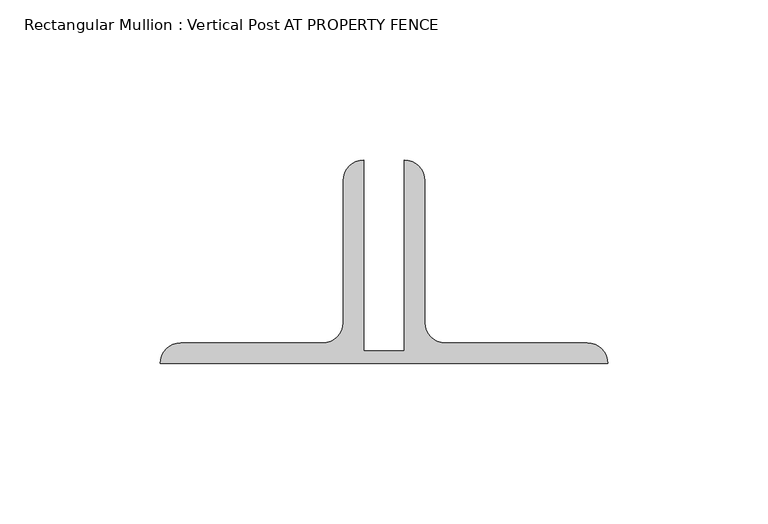
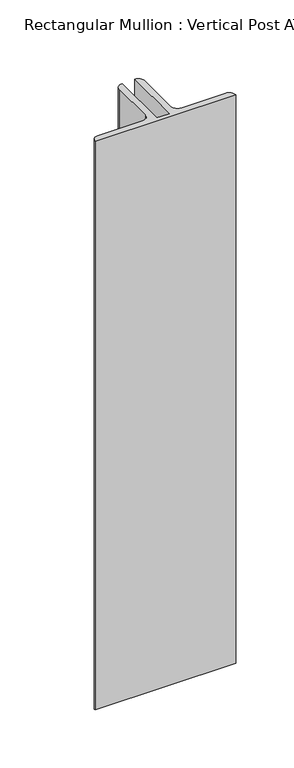
"""IFC4 building model written with IfcOpenShell, lengths in millimetres: member geometry, Rectangular Mullion : Vertical Post AT PROPERTY FENCE."""

import ifcopenshell
import ifcopenshell.guid

model = None  # the IFC model being written
_history = None  # IfcOwnerHistory: only IFC2X3 demands one
_inside = {}  # id of a spatial element -> (the spatial element, [elements in it])
_under = {}  # id of a project, library or spatial element -> (it, [spatial elements below it])
_declared = {}  # id of a project -> (the project, [libraries it declares])
_typed = {}  # id of a type object -> (the type object, [elements of that type])
_made_of = {}  # id of a material, layer set ... -> (it, [elements and type objects made of it])


def new_model(schema):
    """Start an empty IFC model of exactly this schema.

    Asked for "IFC4X3", IfcOpenShell would pick the latest addendum, in which some entities
    have other attributes; the version numbers below select the first issue.
    IFC2X3 requires an IfcOwnerHistory on every rooted entity: one is made here for all.
    """
    global model, _history
    if schema == "IFC4X3":
        model = ifcopenshell.file(schema_version=(4, 3, 0, 0))
    else:
        model = ifcopenshell.file(schema=schema)
    _inside.clear()
    _under.clear()
    _declared.clear()
    _typed.clear()
    _made_of.clear()
    _history = None
    if model.schema == "IFC2X3":
        org = make("IfcOrganization", Name="unknown")
        user = make(
            "IfcPersonAndOrganization",
            ThePerson=make("IfcPerson", FamilyName="unknown"),
            TheOrganization=org,
        )
        app = make(
            "IfcApplication",
            ApplicationDeveloper=org,
            Version="unknown",
            ApplicationFullName="unknown",
            ApplicationIdentifier="unknown",
        )
        _history = make(
            "IfcOwnerHistory",
            OwningUser=user,
            OwningApplication=app,
            ChangeAction="ADDED",
            CreationDate=0,
        )
    return model


def make(cls, **values):
    """One entity of the class cls with the attributes given. An attribute that is None is left unset."""
    return model.create_entity(
        cls, **{name: value for name, value in values.items() if value is not None}
    )


def rooted(cls, **values):
    """An entity with a GlobalId (a new one), such as an element, a storey or a relation."""
    return make(cls, GlobalId=ifcopenshell.guid.new(), OwnerHistory=_history, **values)


def si_unit(unit_type, name, prefix=None):
    """IfcSIUnit, for example si_unit("LENGTHUNIT", "METRE", prefix="MILLI")."""
    return make("IfcSIUnit", UnitType=unit_type, Prefix=prefix, Name=name)


def assignment(units):
    """IfcUnitAssignment: the units of a project."""
    return None if units is None else make("IfcUnitAssignment", Units=units)


def point(xyz):
    """IfcCartesianPoint."""
    return None if xyz is None else make("IfcCartesianPoint", Coordinates=xyz)


def direction(xyz):
    """IfcDirection."""
    return None if xyz is None else make("IfcDirection", DirectionRatios=xyz)


def frame(location, z_axis=None, x_axis=None):
    """IfcAxis2Placement3D, a coordinate frame: its origin and axes. An axis left out is left unset."""
    return make(
        "IfcAxis2Placement3D",
        Location=point(location),
        Axis=direction(z_axis),
        RefDirection=direction(x_axis),
    )


def frame_2d(location, x_axis=None):
    """IfcAxis2Placement2D, a coordinate frame in the plane: its origin and x axis."""
    return make(
        "IfcAxis2Placement2D", Location=point(location), RefDirection=direction(x_axis)
    )


def origin():
    """The frame at (0, 0, 0) with its axes left unset."""
    return frame((0.0, 0.0, 0.0))


def place(relative_to, where):
    """IfcLocalPlacement: puts the frame where relative to a parent placement (None: the world)."""
    return make(
        "IfcLocalPlacement", PlacementRelTo=relative_to, RelativePlacement=where
    )


def context(
    kind, dimensions, precision=None, world=None, true_north=None, identifier=None
):
    """IfcGeometricRepresentationContext, for example the 3D "Model" context."""
    return make(
        "IfcGeometricRepresentationContext",
        ContextIdentifier=identifier,
        ContextType=kind,
        CoordinateSpaceDimension=dimensions,
        Precision=precision,
        WorldCoordinateSystem=world,
        TrueNorth=true_north,
    )


def project(units=None, contexts=None):
    """IfcProject with its units and contexts."""
    return rooted(
        "IfcProject",
        Name="project",
        RepresentationContexts=contexts,
        UnitsInContext=assignment(units),
    )


def spatial(cls, under=None, at=None, **own):
    """A site, building, storey or space (cls), placed at a placement, below another one or the project."""
    s = rooted(cls, ObjectPlacement=at, **own)
    if under is not None:
        _under.setdefault(under.id(), (under, []))[1].append(s)
    return s


def polyline(points):
    """IfcPolyline through the points."""
    return make("IfcPolyline", Points=[point(p) for p in points])


def circle_curve(where, radius):
    """IfcCircle in the frame where."""
    return make("IfcCircle", Position=where, Radius=radius)


def trimmed(basis, trim1, trim2, sense, master):
    """IfcTrimmedCurve: the piece of a basis curve between two trims."""
    return make(
        "IfcTrimmedCurve",
        BasisCurve=basis,
        Trim1=trim1,
        Trim2=trim2,
        SenseAgreement=sense,
        MasterRepresentation=master,
    )


def segment(curve, same_sense, transition):
    """IfcCompositeCurveSegment."""
    return make(
        "IfcCompositeCurveSegment",
        Transition=transition,
        SameSense=same_sense,
        ParentCurve=curve,
    )


def composite_curve(segments, self_intersect=None):
    """IfcCompositeCurve: segments joined end to end."""
    return make("IfcCompositeCurve", Segments=segments, SelfIntersect=self_intersect)


def outline(outer, holes=None, kind="AREA"):
    """IfcArbitraryClosedProfileDef: a profile drawn as a closed curve; with holes, ...WithVoids."""
    if holes is None:
        return make("IfcArbitraryClosedProfileDef", ProfileType=kind, OuterCurve=outer)
    return make(
        "IfcArbitraryProfileDefWithVoids",
        ProfileType=kind,
        OuterCurve=outer,
        InnerCurves=holes,
    )


def extrude(swept, where, along, depth):
    """IfcExtrudedAreaSolid: the profile swept, set in the frame where, extruded along a direction by depth."""
    return make(
        "IfcExtrudedAreaSolid",
        SweptArea=swept,
        Position=where,
        ExtrudedDirection=direction(along),
        Depth=depth,
    )


def shape(context_of_items, identifier, shape_type, items):
    """IfcShapeRepresentation: the items that make up one representation, for example the "Body"."""
    return make(
        "IfcShapeRepresentation",
        ContextOfItems=context_of_items,
        RepresentationIdentifier=identifier,
        RepresentationType=shape_type,
        Items=items,
    )


def source(mapping_origin, context_of_items, identifier, shape_type, items):
    """IfcRepresentationMap: a shape defined once, which mapped items show again and again."""
    return make(
        "IfcRepresentationMap",
        MappingOrigin=mapping_origin,
        MappedRepresentation=shape(context_of_items, identifier, shape_type, items),
    )


def transform(
    local_origin,
    x_axis=None,
    y_axis=None,
    z_axis=None,
    scale=None,
    scale2=None,
    scale3=None,
    uniform=True,
):
    """IfcCartesianTransformationOperator3D, or its non-uniform kind. x_axis, y_axis, z_axis: its Axis1, 2, 3."""
    if uniform:
        return make(
            "IfcCartesianTransformationOperator3D",
            Axis1=direction(x_axis),
            Axis2=direction(y_axis),
            LocalOrigin=point(local_origin),
            Scale=scale,
            Axis3=direction(z_axis),
        )
    return make(
        "IfcCartesianTransformationOperator3DnonUniform",
        Axis1=direction(x_axis),
        Axis2=direction(y_axis),
        LocalOrigin=point(local_origin),
        Scale=scale,
        Axis3=direction(z_axis),
        Scale2=scale2,
        Scale3=scale3,
    )


def mapped(mapping_source, mapping_target):
    """IfcMappedItem: shows the shape of a source again, moved by a transform."""
    return make(
        "IfcMappedItem", MappingSource=mapping_source, MappingTarget=mapping_target
    )


def made_of(thing, what):
    """Note that an element or type object is made of a material, layer set ...; save() writes the relation."""
    if what is not None:
        _made_of.setdefault(what.id(), (what, []))[1].append(thing)
    return thing


def element(
    cls,
    number,
    at=None,
    inside=None,
    cuts=None,
    type_object=None,
    material=None,
    context=None,
    identifier="Body",
    shape_type=None,
    held_by="IfcProductDefinitionShape",
    body=None,
    shapes=None,
    **own,
):
    """One element of the class cls, such as IfcWall. Its Tag is "e" and its number.

    at: its placement. inside: the storey or other place that contains it. cuts: it is an
    opening in that element (IfcRelVoidsElement). A single representation is given by context,
    identifier, shape_type and body (its items); several are given by shapes. held_by: the class
    of the entity that holds the representations. save() writes the other relations.
    """
    e = rooted(cls, Tag="e%d" % number, ObjectPlacement=at, **own)
    if body is not None:
        shapes = [shape(context, identifier, shape_type, body)]
    if shapes is not None:
        e.Representation = make(held_by, Representations=shapes)
    if inside is not None:
        _inside.setdefault(inside.id(), (inside, []))[1].append(e)
    if cuts is not None:
        rooted(
            "IfcRelVoidsElement", RelatingBuildingElement=cuts, RelatedOpeningElement=e
        )
    if type_object is not None:
        _typed.setdefault(type_object.id(), (type_object, []))[1].append(e)
    return made_of(e, material)


def aggregate(whole, parts):
    """IfcRelAggregates: a whole, such as a stair, and the parts it consists of."""
    return rooted("IfcRelAggregates", RelatingObject=whole, RelatedObjects=parts)


def save(model, path):
    """Write the relations noted so far, then the file.

    IfcRelAggregates (storeys below a building ...), IfcRelContainedInSpatialStructure (elements
    in a storey), IfcRelDefinesByType, IfcRelAssociatesMaterial and IfcRelDeclares: one each for
    every whole, place, type object, material and project.
    """
    for whole, parts in _under.values():
        aggregate(whole, parts)
    for where, things in _inside.values():
        rooted(
            "IfcRelContainedInSpatialStructure",
            RelatedElements=things,
            RelatingStructure=where,
        )
    for kind, things in _typed.values():
        rooted("IfcRelDefinesByType", RelatedObjects=things, RelatingType=kind)
    for what, things in _made_of.values():
        rooted("IfcRelAssociatesMaterial", RelatedObjects=things, RelatingMaterial=what)
    for by, libraries in _declared.values():
        rooted("IfcRelDeclares", RelatingContext=by, RelatedDefinitions=libraries)
    model.write(path)


def rectangular_mullion_vertical_post_at_property_fence_f660218a(model_context):
    return source(origin(), model_context, "Body", "SweptSolid", [
        extrude(outline(composite_curve([segment(polyline([(-76.2, 22.9145205), (-63.5, 22.9145205), (-63.5, 82.55)]), True, "CONTINUOUS"), segment(trimmed(circle_curve(frame_2d((-63.5, 76.2)), 6.35), [point((-63.5, 82.55))], [point((-57.15, 76.2))], False, "CARTESIAN"), True, "CONTINUOUS"), segment(polyline([(-57.15, 76.2), (-57.15, 31.75)]), True, "CONTINUOUS"), segment(trimmed(circle_curve(frame_2d((-50.8, 31.75)), 6.35), [point((-57.15, 31.75))], [point((-50.8, 25.4))], True, "CARTESIAN"), True, "CONTINUOUS"), segment(polyline([(-50.8, 25.4), (-6.35, 25.4)]), True, "CONTINUOUS"), segment(trimmed(circle_curve(frame_2d((-6.35, 19.05)), 6.35), [point((-6.35, 25.4))], [point((0.0, 19.05))], False, "CARTESIAN"), True, "CONTINUOUS"), segment(polyline([(0.0, 19.05), (-139.7, 19.05)]), True, "CONTINUOUS"), segment(trimmed(circle_curve(frame_2d((-133.35, 19.05)), 6.35), [point((-139.7, 19.05))], [point((-133.35, 25.4))], False, "CARTESIAN"), True, "CONTINUOUS"), segment(polyline([(-133.35, 25.4), (-88.9, 25.4)]), True, "CONTINUOUS"), segment(trimmed(circle_curve(frame_2d((-88.9, 31.75)), 6.35), [point((-88.9, 25.4))], [point((-82.55, 31.75))], True, "CARTESIAN"), True, "CONTINUOUS"), segment(polyline([(-82.55, 31.75), (-82.55, 76.2)]), True, "CONTINUOUS"), segment(trimmed(circle_curve(frame_2d((-76.2, 76.2)), 6.35), [point((-82.55, 76.2))], [point((-76.2, 82.55))], False, "CARTESIAN"), True, "CONTINUOUS"), segment(polyline([(-76.2, 82.55), (-76.2, 22.9145205)]), True, "CONTINUOUS")], self_intersect=False)), frame((0.0, 0.0, -596.9), z_axis=(0.0, 0.0, 1.0), x_axis=(1.0, 0.0, 0.0)), (0.0, 0.0, 1.0), 596.9),
    ])


if __name__ == "__main__":
    model = new_model("IFC4")
    model_context = context("Model", 3, world=origin())
    ifc_project = project(units=[si_unit("LENGTHUNIT", "METRE", prefix="MILLI")], contexts=[model_context])
    site = spatial("IfcSite", under=ifc_project)
    building = spatial("IfcBuilding", under=site)
    placement = place(None, origin())
    rectangular_mullion_vertical_post_at_property_fence_shape = rectangular_mullion_vertical_post_at_property_fence_f660218a(model_context)
    element("IfcMember", 1, ObjectType="Rectangular Mullion : Vertical Post AT PROPERTY FENCE", at=placement, inside=building, context=model_context, shape_type="MappedRepresentation", body=[
        mapped(rectangular_mullion_vertical_post_at_property_fence_shape, transform((0.0, 0.0, 0.0), x_axis=(1.0, 0.0, 0.0), y_axis=(0.0, 1.0, 0.0), z_axis=(0.0, 0.0, 1.0))),
    ])
    save(model, "model.ifc")

# Revit data of these elements
# Type "Rectangular Mullion : Vertical Post AT PROPERTY FENCE"
#   built-in parameter 1007351 = -0.0625 (stored number, unit not read)
#   built-in parameter 1007322 = 0.0126789 (stored number, unit not read)
#   built-in parameter 1007321 = 0.229167 (stored number, unit not read)
#   built-in parameter 1007320 = 0.229167 (stored number, unit not read)
# Element 1 (IfcMember, "Rectangular Mullion : Vertical Post AT PROPERTY FENCE")
#   Materials on its faces: "MAIN FENCE POST: (2) BACK/BACK GALVANIZED ANGLES (2) L2 1/2 X 2 1/2 X 1/4\") ANCHORED TO 8\"W X 42\" DEEP CONCRETE FOOTING(1)"
# Materials
#   "MAIN FENCE POST: (2) BACK/BACK GALVANIZED ANGLES (2) L2 1/2 X 2 1/2 X 1/4\") ANCHORED TO 8\"W X 42\" DEEP CONCRETE FOOTING(1)": class "Unassigned", colour RGB 211 211 211, transparency 0, Cost = 0
